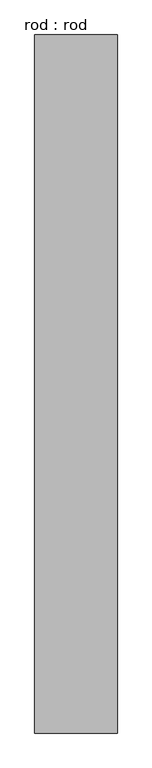
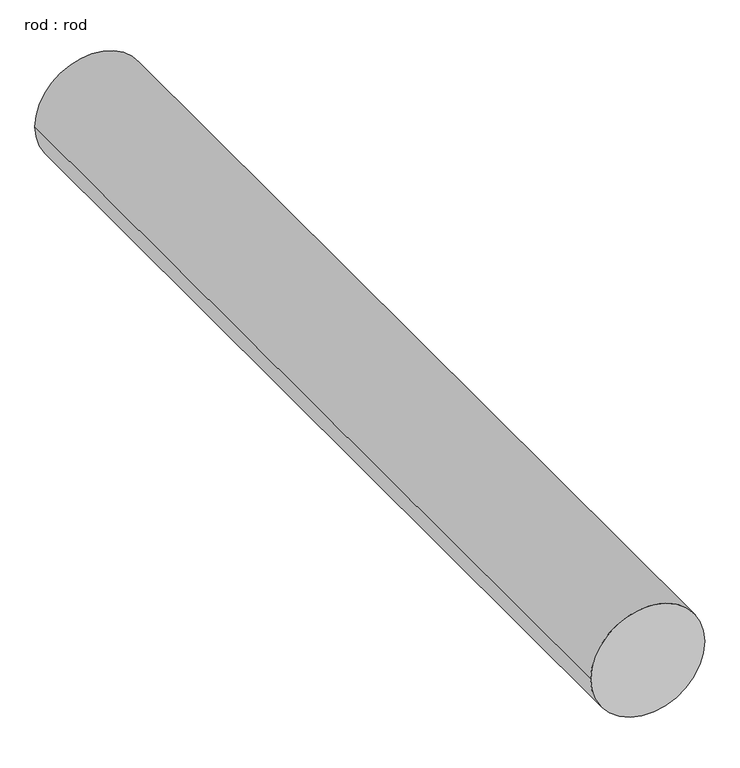
"""IFC4 building model written with IfcOpenShell, lengths in millimetres: proxy geometry, rod : rod."""

from ifc_helpers import new_model, si_unit, point, frame, frame_2d, origin, place, context, project, spatial, circle_curve, trimmed, segment, composite_curve, outline, extrude, source, transform, mapped, element, save


def rod_rod_3bf34879(model_context):
    return source(origin(), model_context, "Body", "SweptSolid", [
        extrude(outline(composite_curve([segment(trimmed(circle_curve(frame_2d((0.0108462, 0.0)), 200.0), [point((0.0108462, 200.0))], [point((0.0108462, -200.0))], False, "CARTESIAN"), True, "CONTINUOUS"), segment(trimmed(circle_curve(frame_2d((0.0108462, 0.0)), 200.0), [point((0.0108462, -200.0))], [point((0.0108462, 200.0))], False, "CARTESIAN"), True, "CONTINUOUS")], self_intersect=False)), frame((0.0, 2402.7286153, 0.0), z_axis=(0.0, 1.0, 0.0), x_axis=(0.0, 0.0, 1.0)), (0.0, 0.0, 1.0), 3380.0),
    ])


if __name__ == "__main__":
    model = new_model("IFC4")
    model_context = context("Model", 3, world=origin())
    ifc_project = project(units=[si_unit("LENGTHUNIT", "METRE", prefix="MILLI")], contexts=[model_context])
    site = spatial("IfcSite", under=ifc_project)
    building = spatial("IfcBuilding", under=site)
    placement = place(None, origin())
    rod_rod_shape = rod_rod_3bf34879(model_context)
    element("IfcBuildingElementProxy", 1, Name="rod : rod", ObjectType="rod : rod", at=placement, inside=building, context=model_context, shape_type="MappedRepresentation", body=[
        mapped(rod_rod_shape, transform((0.0, 0.0, 0.0), x_axis=(1.0, 0.0, 0.0), y_axis=(0.0, 1.0, 0.0), z_axis=(0.0, 0.0, 1.0))),
    ])
    save(model, "model.ifc")

# Revit data of these elements
# Type "rod : rod"
#   Default Elevation = 0
